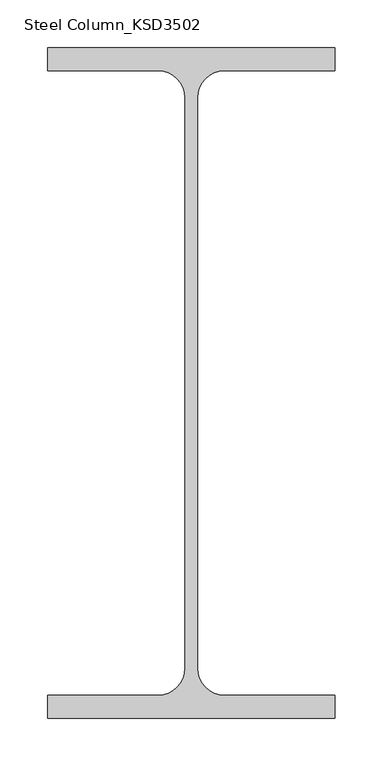
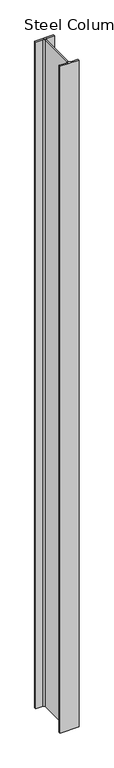
"""IFC4 building model written with IfcOpenShell, lengths in millimetres: column geometry, Steel Column_KSD3502 : H_SC_ASC_H-700×300x13x24."""

import ifcopenshell
import ifcopenshell.guid

model = None  # the IFC model being written
_history = None  # IfcOwnerHistory: only IFC2X3 demands one
_inside = {}  # id of a spatial element -> (the spatial element, [elements in it])
_under = {}  # id of a project, library or spatial element -> (it, [spatial elements below it])
_declared = {}  # id of a project -> (the project, [libraries it declares])
_typed = {}  # id of a type object -> (the type object, [elements of that type])
_made_of = {}  # id of a material, layer set ... -> (it, [elements and type objects made of it])


def new_model(schema):
    """Start an empty IFC model of exactly this schema.

    Asked for "IFC4X3", IfcOpenShell would pick the latest addendum, in which some entities
    have other attributes; the version numbers below select the first issue.
    IFC2X3 requires an IfcOwnerHistory on every rooted entity: one is made here for all.
    """
    global model, _history
    if schema == "IFC4X3":
        model = ifcopenshell.file(schema_version=(4, 3, 0, 0))
    else:
        model = ifcopenshell.file(schema=schema)
    _inside.clear()
    _under.clear()
    _declared.clear()
    _typed.clear()
    _made_of.clear()
    _history = None
    if model.schema == "IFC2X3":
        org = make("IfcOrganization", Name="unknown")
        user = make(
            "IfcPersonAndOrganization",
            ThePerson=make("IfcPerson", FamilyName="unknown"),
            TheOrganization=org,
        )
        app = make(
            "IfcApplication",
            ApplicationDeveloper=org,
            Version="unknown",
            ApplicationFullName="unknown",
            ApplicationIdentifier="unknown",
        )
        _history = make(
            "IfcOwnerHistory",
            OwningUser=user,
            OwningApplication=app,
            ChangeAction="ADDED",
            CreationDate=0,
        )
    return model


def make(cls, **values):
    """One entity of the class cls with the attributes given. An attribute that is None is left unset."""
    return model.create_entity(
        cls, **{name: value for name, value in values.items() if value is not None}
    )


def rooted(cls, **values):
    """An entity with a GlobalId (a new one), such as an element, a storey or a relation."""
    return make(cls, GlobalId=ifcopenshell.guid.new(), OwnerHistory=_history, **values)


def si_unit(unit_type, name, prefix=None):
    """IfcSIUnit, for example si_unit("LENGTHUNIT", "METRE", prefix="MILLI")."""
    return make("IfcSIUnit", UnitType=unit_type, Prefix=prefix, Name=name)


def assignment(units):
    """IfcUnitAssignment: the units of a project."""
    return None if units is None else make("IfcUnitAssignment", Units=units)


def point(xyz):
    """IfcCartesianPoint."""
    return None if xyz is None else make("IfcCartesianPoint", Coordinates=xyz)


def direction(xyz):
    """IfcDirection."""
    return None if xyz is None else make("IfcDirection", DirectionRatios=xyz)


def frame(location, z_axis=None, x_axis=None):
    """IfcAxis2Placement3D, a coordinate frame: its origin and axes. An axis left out is left unset."""
    return make(
        "IfcAxis2Placement3D",
        Location=point(location),
        Axis=direction(z_axis),
        RefDirection=direction(x_axis),
    )


def frame_2d(location, x_axis=None):
    """IfcAxis2Placement2D, a coordinate frame in the plane: its origin and x axis."""
    return make(
        "IfcAxis2Placement2D", Location=point(location), RefDirection=direction(x_axis)
    )


def origin():
    """The frame at (0, 0, 0) with its axes left unset."""
    return frame((0.0, 0.0, 0.0))


def place(relative_to, where):
    """IfcLocalPlacement: puts the frame where relative to a parent placement (None: the world)."""
    return make(
        "IfcLocalPlacement", PlacementRelTo=relative_to, RelativePlacement=where
    )


def context(
    kind, dimensions, precision=None, world=None, true_north=None, identifier=None
):
    """IfcGeometricRepresentationContext, for example the 3D "Model" context."""
    return make(
        "IfcGeometricRepresentationContext",
        ContextIdentifier=identifier,
        ContextType=kind,
        CoordinateSpaceDimension=dimensions,
        Precision=precision,
        WorldCoordinateSystem=world,
        TrueNorth=true_north,
    )


def project(units=None, contexts=None):
    """IfcProject with its units and contexts."""
    return rooted(
        "IfcProject",
        Name="project",
        RepresentationContexts=contexts,
        UnitsInContext=assignment(units),
    )


def spatial(cls, under=None, at=None, **own):
    """A site, building, storey or space (cls), placed at a placement, below another one or the project."""
    s = rooted(cls, ObjectPlacement=at, **own)
    if under is not None:
        _under.setdefault(under.id(), (under, []))[1].append(s)
    return s


def polyline(points):
    """IfcPolyline through the points."""
    return make("IfcPolyline", Points=[point(p) for p in points])


def circle_curve(where, radius):
    """IfcCircle in the frame where."""
    return make("IfcCircle", Position=where, Radius=radius)


def trimmed(basis, trim1, trim2, sense, master):
    """IfcTrimmedCurve: the piece of a basis curve between two trims."""
    return make(
        "IfcTrimmedCurve",
        BasisCurve=basis,
        Trim1=trim1,
        Trim2=trim2,
        SenseAgreement=sense,
        MasterRepresentation=master,
    )


def segment(curve, same_sense, transition):
    """IfcCompositeCurveSegment."""
    return make(
        "IfcCompositeCurveSegment",
        Transition=transition,
        SameSense=same_sense,
        ParentCurve=curve,
    )


def composite_curve(segments, self_intersect=None):
    """IfcCompositeCurve: segments joined end to end."""
    return make("IfcCompositeCurve", Segments=segments, SelfIntersect=self_intersect)


def outline(outer, holes=None, kind="AREA"):
    """IfcArbitraryClosedProfileDef: a profile drawn as a closed curve; with holes, ...WithVoids."""
    if holes is None:
        return make("IfcArbitraryClosedProfileDef", ProfileType=kind, OuterCurve=outer)
    return make(
        "IfcArbitraryProfileDefWithVoids",
        ProfileType=kind,
        OuterCurve=outer,
        InnerCurves=holes,
    )


def extrude(swept, where, along, depth):
    """IfcExtrudedAreaSolid: the profile swept, set in the frame where, extruded along a direction by depth."""
    return make(
        "IfcExtrudedAreaSolid",
        SweptArea=swept,
        Position=where,
        ExtrudedDirection=direction(along),
        Depth=depth,
    )


def shape(context_of_items, identifier, shape_type, items):
    """IfcShapeRepresentation: the items that make up one representation, for example the "Body"."""
    return make(
        "IfcShapeRepresentation",
        ContextOfItems=context_of_items,
        RepresentationIdentifier=identifier,
        RepresentationType=shape_type,
        Items=items,
    )


def source(mapping_origin, context_of_items, identifier, shape_type, items):
    """IfcRepresentationMap: a shape defined once, which mapped items show again and again."""
    return make(
        "IfcRepresentationMap",
        MappingOrigin=mapping_origin,
        MappedRepresentation=shape(context_of_items, identifier, shape_type, items),
    )


def transform(
    local_origin,
    x_axis=None,
    y_axis=None,
    z_axis=None,
    scale=None,
    scale2=None,
    scale3=None,
    uniform=True,
):
    """IfcCartesianTransformationOperator3D, or its non-uniform kind. x_axis, y_axis, z_axis: its Axis1, 2, 3."""
    if uniform:
        return make(
            "IfcCartesianTransformationOperator3D",
            Axis1=direction(x_axis),
            Axis2=direction(y_axis),
            LocalOrigin=point(local_origin),
            Scale=scale,
            Axis3=direction(z_axis),
        )
    return make(
        "IfcCartesianTransformationOperator3DnonUniform",
        Axis1=direction(x_axis),
        Axis2=direction(y_axis),
        LocalOrigin=point(local_origin),
        Scale=scale,
        Axis3=direction(z_axis),
        Scale2=scale2,
        Scale3=scale3,
    )


def mapped(mapping_source, mapping_target):
    """IfcMappedItem: shows the shape of a source again, moved by a transform."""
    return make(
        "IfcMappedItem", MappingSource=mapping_source, MappingTarget=mapping_target
    )


def made_of(thing, what):
    """Note that an element or type object is made of a material, layer set ...; save() writes the relation."""
    if what is not None:
        _made_of.setdefault(what.id(), (what, []))[1].append(thing)
    return thing


def element(
    cls,
    number,
    at=None,
    inside=None,
    cuts=None,
    type_object=None,
    material=None,
    context=None,
    identifier="Body",
    shape_type=None,
    held_by="IfcProductDefinitionShape",
    body=None,
    shapes=None,
    **own,
):
    """One element of the class cls, such as IfcWall. Its Tag is "e" and its number.

    at: its placement. inside: the storey or other place that contains it. cuts: it is an
    opening in that element (IfcRelVoidsElement). A single representation is given by context,
    identifier, shape_type and body (its items); several are given by shapes. held_by: the class
    of the entity that holds the representations. save() writes the other relations.
    """
    e = rooted(cls, Tag="e%d" % number, ObjectPlacement=at, **own)
    if body is not None:
        shapes = [shape(context, identifier, shape_type, body)]
    if shapes is not None:
        e.Representation = make(held_by, Representations=shapes)
    if inside is not None:
        _inside.setdefault(inside.id(), (inside, []))[1].append(e)
    if cuts is not None:
        rooted(
            "IfcRelVoidsElement", RelatingBuildingElement=cuts, RelatedOpeningElement=e
        )
    if type_object is not None:
        _typed.setdefault(type_object.id(), (type_object, []))[1].append(e)
    return made_of(e, material)


def aggregate(whole, parts):
    """IfcRelAggregates: a whole, such as a stair, and the parts it consists of."""
    return rooted("IfcRelAggregates", RelatingObject=whole, RelatedObjects=parts)


def save(model, path):
    """Write the relations noted so far, then the file.

    IfcRelAggregates (storeys below a building ...), IfcRelContainedInSpatialStructure (elements
    in a storey), IfcRelDefinesByType, IfcRelAssociatesMaterial and IfcRelDeclares: one each for
    every whole, place, type object, material and project.
    """
    for whole, parts in _under.values():
        aggregate(whole, parts)
    for where, things in _inside.values():
        rooted(
            "IfcRelContainedInSpatialStructure",
            RelatedElements=things,
            RelatingStructure=where,
        )
    for kind, things in _typed.values():
        rooted("IfcRelDefinesByType", RelatedObjects=things, RelatingType=kind)
    for what, things in _made_of.values():
        rooted("IfcRelAssociatesMaterial", RelatedObjects=things, RelatingMaterial=what)
    for by, libraries in _declared.values():
        rooted("IfcRelDeclares", RelatingContext=by, RelatedDefinitions=libraries)
    model.write(path)


def steel_column_ksd3502_8461dad7(model_context):
    return source(origin(), model_context, "Body", "SweptSolid", [
        extrude(outline(composite_curve([segment(polyline([(150.0, 350.0), (150.0, 326.0), (34.5, 326.0)]), True, "CONTINUOUS"), segment(trimmed(circle_curve(frame_2d((34.5, 298.0)), 28.0), [point((34.5, 326.0))], [point((6.5, 298.0))], True, "CARTESIAN"), True, "CONTINUOUS"), segment(polyline([(6.5, 298.0), (6.5, -298.0)]), True, "CONTINUOUS"), segment(trimmed(circle_curve(frame_2d((34.5, -298.0)), 28.0), [point((6.5, -298.0))], [point((34.5, -326.0))], True, "CARTESIAN"), True, "CONTINUOUS"), segment(polyline([(34.5, -326.0), (150.0, -326.0), (150.0, -350.0), (-150.0, -350.0), (-150.0, -326.0), (-34.5, -326.0)]), True, "CONTINUOUS"), segment(trimmed(circle_curve(frame_2d((-34.5, -298.0)), 28.0), [point((-34.5, -326.0))], [point((-6.5, -298.0))], True, "CARTESIAN"), True, "CONTINUOUS"), segment(polyline([(-6.5, -298.0), (-6.5, 298.0)]), True, "CONTINUOUS"), segment(trimmed(circle_curve(frame_2d((-34.5, 298.0)), 28.0), [point((-6.5, 298.0))], [point((-34.5, 326.0))], True, "CARTESIAN"), True, "CONTINUOUS"), segment(polyline([(-34.5, 326.0), (-150.0, 326.0), (-150.0, 350.0), (150.0, 350.0)]), True, "CONTINUOUS")], self_intersect=False)), frame((0.0, 0.0, 685.9720055), z_axis=(0.0, 0.0, 1.0), x_axis=(1.0, 0.0, 0.0)), (0.0, 0.0, 1.0), 11224.0),
    ])


if __name__ == "__main__":
    model = new_model("IFC4")
    model_context = context("Model", 3, world=origin())
    ifc_project = project(units=[si_unit("LENGTHUNIT", "METRE", prefix="MILLI")], contexts=[model_context])
    site = spatial("IfcSite", under=ifc_project)
    building = spatial("IfcBuilding", under=site)
    placement = place(None, origin())
    steel_column_ksd3502_shape = steel_column_ksd3502_8461dad7(model_context)
    element("IfcColumn", 1, ObjectType="Steel Column_KSD3502 : H_SC_ASC_H-700×300x13x24", at=placement, inside=building, context=model_context, shape_type="MappedRepresentation", body=[
        mapped(steel_column_ksd3502_shape, transform((0.0, 0.0, 0.0), x_axis=(1.0, 0.0, 0.0), y_axis=(0.0, 1.0, 0.0), z_axis=(0.0, 0.0, 1.0))),
    ])
    save(model, "model.ifc")

# Revit data of these elements
# Type "Steel Column_KSD3502 : H_SC_ASC_H-700×300x13x24"
#   Width = 30.0 cm
#   Web Thickness = 1.3 cm
#   Web Fillet = 2.8 cm
#   Warping Constant = 12338400.0 cm⁶
#   Torsional Moment of Inertia = 325.986 cm⁴
#   Section Area = 235.5 cm²
#   Plastic Modulus weak axis = 1120.0 cm³
#   Plastic Modulus strong axis = 6460.0 cm³
#   Perimeter = 1.27 m²/m
#   Nominal Weight = 185.00 kgf/m
#   Moment of Inertia weak axis = 10800.00 cm⁴
#   Moment of Inertia strong axis = 201000.00 cm⁴
#   Height = 70.0 cm
#   Flange Thickness = 2.4 cm
#   Elastic Modulus weak axis = 722.0 cm³
#   Elastic Modulus strong axis = 5760.0 cm³
#   Centroid Vertical = 35.0 cm
#   Centroid Horizontal = 15.0 cm
#   Bolt Spacing = 13.97 cm
#   Structural Material [instance default] = Steel, 45-345
#   Section Name Key = ""
#   Assembly Code = ""
# Element 1 (IfcColumn, "Steel Column_KSD3502 : H_SC_ASC_H-700×300x13x24")
#   Structural Material = A03AD029-00008_Anchor Bolt (Installation only)_M36
#   Materials on its faces: "A03AD029-00008_Anchor Bolt (Installation only)_M36"
# Materials
#   "Steel, 45-345": class "Metal", colour RGB 189 187 185, transparency 0, Description = "Steel 345 MPa", Cost = 0
#   "A03AD029-00008_Anchor Bolt (Installation only)_M36": class "Unassigned", colour RGB 84 83 81, transparency 0, Cost = 0
